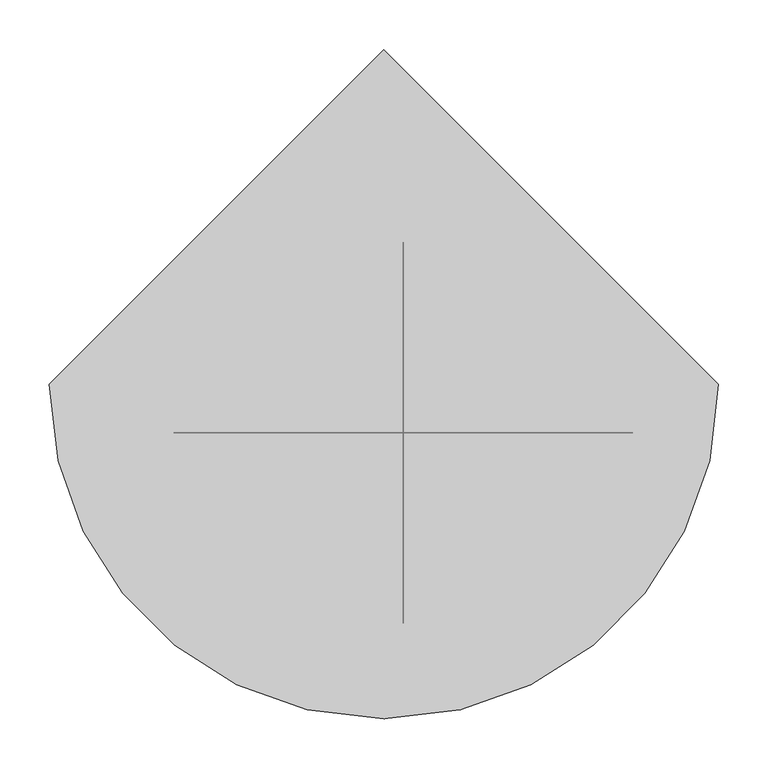
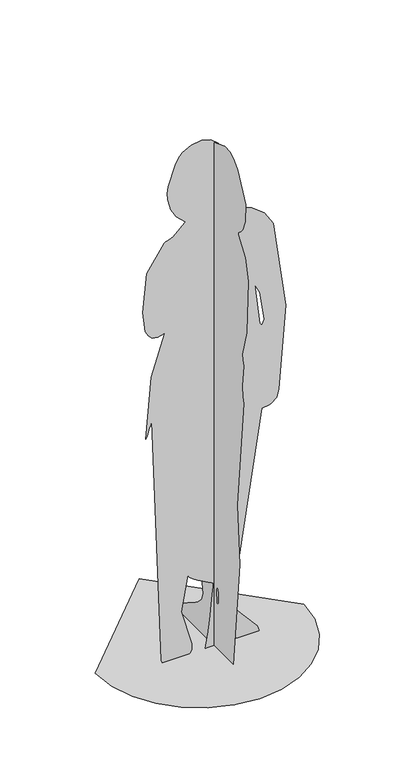
"""IFC4 building model written with IfcOpenShell, lengths in millimetres: proxy geometry, yinyin 25485 : yinyin 25485."""

import ifcopenshell
import ifcopenshell.guid

model = None  # the IFC model being written
_history = None  # IfcOwnerHistory: only IFC2X3 demands one
_inside = {}  # id of a spatial element -> (the spatial element, [elements in it])
_under = {}  # id of a project, library or spatial element -> (it, [spatial elements below it])
_declared = {}  # id of a project -> (the project, [libraries it declares])
_typed = {}  # id of a type object -> (the type object, [elements of that type])
_made_of = {}  # id of a material, layer set ... -> (it, [elements and type objects made of it])


def new_model(schema):
    """Start an empty IFC model of exactly this schema.

    Asked for "IFC4X3", IfcOpenShell would pick the latest addendum, in which some entities
    have other attributes; the version numbers below select the first issue.
    IFC2X3 requires an IfcOwnerHistory on every rooted entity: one is made here for all.
    """
    global model, _history
    if schema == "IFC4X3":
        model = ifcopenshell.file(schema_version=(4, 3, 0, 0))
    else:
        model = ifcopenshell.file(schema=schema)
    _inside.clear()
    _under.clear()
    _declared.clear()
    _typed.clear()
    _made_of.clear()
    _history = None
    if model.schema == "IFC2X3":
        org = make("IfcOrganization", Name="unknown")
        user = make(
            "IfcPersonAndOrganization",
            ThePerson=make("IfcPerson", FamilyName="unknown"),
            TheOrganization=org,
        )
        app = make(
            "IfcApplication",
            ApplicationDeveloper=org,
            Version="unknown",
            ApplicationFullName="unknown",
            ApplicationIdentifier="unknown",
        )
        _history = make(
            "IfcOwnerHistory",
            OwningUser=user,
            OwningApplication=app,
            ChangeAction="ADDED",
            CreationDate=0,
        )
    return model


def make(cls, **values):
    """One entity of the class cls with the attributes given. An attribute that is None is left unset."""
    return model.create_entity(
        cls, **{name: value for name, value in values.items() if value is not None}
    )


def rooted(cls, **values):
    """An entity with a GlobalId (a new one), such as an element, a storey or a relation."""
    return make(cls, GlobalId=ifcopenshell.guid.new(), OwnerHistory=_history, **values)


def si_unit(unit_type, name, prefix=None):
    """IfcSIUnit, for example si_unit("LENGTHUNIT", "METRE", prefix="MILLI")."""
    return make("IfcSIUnit", UnitType=unit_type, Prefix=prefix, Name=name)


def assignment(units):
    """IfcUnitAssignment: the units of a project."""
    return None if units is None else make("IfcUnitAssignment", Units=units)


def point(xyz):
    """IfcCartesianPoint."""
    return None if xyz is None else make("IfcCartesianPoint", Coordinates=xyz)


def direction(xyz):
    """IfcDirection."""
    return None if xyz is None else make("IfcDirection", DirectionRatios=xyz)


def frame(location, z_axis=None, x_axis=None):
    """IfcAxis2Placement3D, a coordinate frame: its origin and axes. An axis left out is left unset."""
    return make(
        "IfcAxis2Placement3D",
        Location=point(location),
        Axis=direction(z_axis),
        RefDirection=direction(x_axis),
    )


def origin():
    """The frame at (0, 0, 0) with its axes left unset."""
    return frame((0.0, 0.0, 0.0))


def place(relative_to, where):
    """IfcLocalPlacement: puts the frame where relative to a parent placement (None: the world)."""
    return make(
        "IfcLocalPlacement", PlacementRelTo=relative_to, RelativePlacement=where
    )


def context(
    kind, dimensions, precision=None, world=None, true_north=None, identifier=None
):
    """IfcGeometricRepresentationContext, for example the 3D "Model" context."""
    return make(
        "IfcGeometricRepresentationContext",
        ContextIdentifier=identifier,
        ContextType=kind,
        CoordinateSpaceDimension=dimensions,
        Precision=precision,
        WorldCoordinateSystem=world,
        TrueNorth=true_north,
    )


def project(units=None, contexts=None):
    """IfcProject with its units and contexts."""
    return rooted(
        "IfcProject",
        Name="project",
        RepresentationContexts=contexts,
        UnitsInContext=assignment(units),
    )


def spatial(cls, under=None, at=None, **own):
    """A site, building, storey or space (cls), placed at a placement, below another one or the project."""
    s = rooted(cls, ObjectPlacement=at, **own)
    if under is not None:
        _under.setdefault(under.id(), (under, []))[1].append(s)
    return s


def point_list(points):
    """IfcCartesianPointList2D or 3D."""
    cls = (
        "IfcCartesianPointList2D" if len(points[0]) == 2 else "IfcCartesianPointList3D"
    )
    return make(cls, CoordList=points)


def triangles(points, corners, closed=None, point_numbers=None):
    """IfcTriangulatedFaceSet: each triangle names its three corners, points numbered from 1."""
    return make(
        "IfcTriangulatedFaceSet",
        Coordinates=point_list(points),
        Closed=closed,
        CoordIndex=corners,
        PnIndex=point_numbers,
    )


def shape(context_of_items, identifier, shape_type, items):
    """IfcShapeRepresentation: the items that make up one representation, for example the "Body"."""
    return make(
        "IfcShapeRepresentation",
        ContextOfItems=context_of_items,
        RepresentationIdentifier=identifier,
        RepresentationType=shape_type,
        Items=items,
    )


def source(mapping_origin, context_of_items, identifier, shape_type, items):
    """IfcRepresentationMap: a shape defined once, which mapped items show again and again."""
    return make(
        "IfcRepresentationMap",
        MappingOrigin=mapping_origin,
        MappedRepresentation=shape(context_of_items, identifier, shape_type, items),
    )


def transform(
    local_origin,
    x_axis=None,
    y_axis=None,
    z_axis=None,
    scale=None,
    scale2=None,
    scale3=None,
    uniform=True,
):
    """IfcCartesianTransformationOperator3D, or its non-uniform kind. x_axis, y_axis, z_axis: its Axis1, 2, 3."""
    if uniform:
        return make(
            "IfcCartesianTransformationOperator3D",
            Axis1=direction(x_axis),
            Axis2=direction(y_axis),
            LocalOrigin=point(local_origin),
            Scale=scale,
            Axis3=direction(z_axis),
        )
    return make(
        "IfcCartesianTransformationOperator3DnonUniform",
        Axis1=direction(x_axis),
        Axis2=direction(y_axis),
        LocalOrigin=point(local_origin),
        Scale=scale,
        Axis3=direction(z_axis),
        Scale2=scale2,
        Scale3=scale3,
    )


def mapped(mapping_source, mapping_target):
    """IfcMappedItem: shows the shape of a source again, moved by a transform."""
    return make(
        "IfcMappedItem", MappingSource=mapping_source, MappingTarget=mapping_target
    )


def made_of(thing, what):
    """Note that an element or type object is made of a material, layer set ...; save() writes the relation."""
    if what is not None:
        _made_of.setdefault(what.id(), (what, []))[1].append(thing)
    return thing


def element(
    cls,
    number,
    at=None,
    inside=None,
    cuts=None,
    type_object=None,
    material=None,
    context=None,
    identifier="Body",
    shape_type=None,
    held_by="IfcProductDefinitionShape",
    body=None,
    shapes=None,
    **own,
):
    """One element of the class cls, such as IfcWall. Its Tag is "e" and its number.

    at: its placement. inside: the storey or other place that contains it. cuts: it is an
    opening in that element (IfcRelVoidsElement). A single representation is given by context,
    identifier, shape_type and body (its items); several are given by shapes. held_by: the class
    of the entity that holds the representations. save() writes the other relations.
    """
    e = rooted(cls, Tag="e%d" % number, ObjectPlacement=at, **own)
    if body is not None:
        shapes = [shape(context, identifier, shape_type, body)]
    if shapes is not None:
        e.Representation = make(held_by, Representations=shapes)
    if inside is not None:
        _inside.setdefault(inside.id(), (inside, []))[1].append(e)
    if cuts is not None:
        rooted(
            "IfcRelVoidsElement", RelatingBuildingElement=cuts, RelatedOpeningElement=e
        )
    if type_object is not None:
        _typed.setdefault(type_object.id(), (type_object, []))[1].append(e)
    return made_of(e, material)


def aggregate(whole, parts):
    """IfcRelAggregates: a whole, such as a stair, and the parts it consists of."""
    return rooted("IfcRelAggregates", RelatingObject=whole, RelatedObjects=parts)


def save(model, path):
    """Write the relations noted so far, then the file.

    IfcRelAggregates (storeys below a building ...), IfcRelContainedInSpatialStructure (elements
    in a storey), IfcRelDefinesByType, IfcRelAssociatesMaterial and IfcRelDeclares: one each for
    every whole, place, type object, material and project.
    """
    for whole, parts in _under.values():
        aggregate(whole, parts)
    for where, things in _inside.values():
        rooted(
            "IfcRelContainedInSpatialStructure",
            RelatedElements=things,
            RelatingStructure=where,
        )
    for kind, things in _typed.values():
        rooted("IfcRelDefinesByType", RelatedObjects=things, RelatingType=kind)
    for what, things in _made_of.values():
        rooted("IfcRelAssociatesMaterial", RelatedObjects=things, RelatingMaterial=what)
    for by, libraries in _declared.values():
        rooted("IfcRelDeclares", RelatingContext=by, RelatedDefinitions=libraries)
    model.write(path)


def entourage_2a7e0e44(model_context):
    return source(origin(), model_context, "Body", "Tessellation", [
        triangles([(19.5612288, -62.516115, 200.054177), (19.5612288, -65.6147495, 206.6420561), (19.5612288, -67.0928433, 208.6188795), (19.5612265, -68.5512254, 210.1580661), (19.5612265, -69.844524, 211.0626257), (19.5612265, -70.8273447, 211.135768), (19.5612265, -72.3676622, 205.9018034), (19.5612265, -74.2961918, 196.3806185), (19.5612265, -75.9136394, 184.6084991), (19.5612265, -76.5207017, 172.6210404), (19.5612265, -75.4180619, 162.4544372), (19.5612265, -71.9064394, 156.1446297), (19.5612288, -65.2864992, 155.7276494), (19.561222, -157.7734002, 0.0), (19.5612197, -193.0714818, 365.6725562), (19.5612197, -178.8732388, 562.9772644), (19.5612197, -217.6589527, 934.2117268), (19.5612197, -211.3346658, 953.6969473), (19.5612197, -209.2266004, 990.3578636), (19.5612197, -217.6589527, 1061.6503143), (19.5612197, -210.505792, 1080.5146425), (19.5612197, -208.859072, 1098.4551172), (19.5612174, -232.5499224, 1186.4916767), (19.5612174, -242.5926415, 1369.1652649), (19.5612197, -225.9702005, 1441.195752), (19.5612197, -184.4141614, 1493.8335274), (19.5612197, -184.4141614, 1502.144648), (19.5612197, -199.7089946, 1513.6221451), (19.5612197, -211.0344297, 1528.1208241), (19.5612197, -224.1337755, 1563.6801361), (19.5612197, -228.7406891, 1624.0425854), (19.5612197, -183.90509, 1715.3903526), (19.561222, -164.1470301, 1737.5990261), (19.561222, -139.3701631, 1750.94981), (19.5612242, -108.0070247, 1752.6), (19.5612288, -48.1992019, 1729.3935677), (19.5612288, -20.4396227, 1708.5970173), (19.5612288, -13.3298936, 1699.5173389), (19.5612288, -7.8875699, 1689.0607098), (19.5612288, -0.7000028, 1662.8370197), (19.5612288, -20.3543195, 1513.0532845), (19.5612288, -18.6669849, 1499.3218552), (19.5612288, 11.1308794, 1439.5698338), (19.5612311, 14.5355749, 1426.8243908), (19.5612288, 1.7224977, 1354.8805264), (19.5612311, 31.6774996, 1150.3032606), (19.5612333, 48.2999633, 1147.5328629), (19.5612333, 62.8445879, 962.6950172), (19.5612356, 95.3969115, 840.0179123), (19.5612356, 94.2716259, 840.4783493), (19.5612356, 92.0029507, 841.6656315), (19.5612356, 89.0270695, 843.2890789), (19.5612356, 85.780102, 845.057939), (19.5612356, 82.698268, 846.6813864), (19.5612356, 80.2176599, 847.8687412), (19.5612356, 78.7744431, 848.3291056), (19.5612379, 129.4411089, 519.2575856), (19.5612356, 115.741936, 386.017608), (19.5612356, 111.0111655, 373.0374773), (19.5612333, 46.365393, 289.3376807), (19.5612311, 27.5485274, 242.7219941), (19.5612288, 11.1591606, 141.8756606), (19.5612311, 19.6101607, 117.1299145), (19.5612311, 40.4985227, 95.464113), (19.5612333, 68.4630586, 75.9257889), (19.5612356, 98.1425106, 57.5627155), (19.5612379, 124.1758143, 39.4220441), (19.5612379, 141.2016192, 20.5520522), (19.5612379, 143.8588244, 0.0), (183.0152098, -49.3669449, 1064.4207121), (167.6047769, -49.3669449, 1163.5493271), (152.5406528, -49.3669449, 1194.6297701), (168.2882199, -49.3669449, 1056.0085802), (175.1435972, -49.3669449, 1046.9906713), (-8.6639288, -49.3669495, 0.0), (-3.1500451, -49.3669495, 32.2482746), (2.0823084, -49.3669495, 69.3733591), (6.8265455, -49.3669495, 108.190362), (10.8761212, -49.3669495, 145.5140468), (14.0244233, -49.3669495, 178.1596922), (16.064901, -49.3669495, 202.9421185), (16.790965, -49.3669495, 216.6765999), (12.1870877, -49.3669495, 219.1461257), (0.3139176, -49.3669495, 225.0791757), (-15.9208339, -49.3669495, 233.4869473), (-33.6094311, -49.3669495, 243.3801843), (-49.8441732, -49.3669495, 253.770157), (-61.7173402, -49.3669495, 263.6679903), (-66.3212244, -49.3669495, 272.0846822), (-87.4455254, -49.3669495, 152.9572698), (-53.4087358, -49.3669495, 31.0045278), (-52.5813699, -49.3669495, 11.0292914), (-59.149233, -49.3669495, 0.0), (-149.3170486, -49.3669495, 0.0), (-152.8115664, -49.3669495, 10.4443548), (-182.6783299, -49.3669495, 842.7883101), (-184.325068, -49.3669495, 839.6736019), (-187.3181266, -49.3669495, 831.6521439), (-191.0743654, -49.3669495, 820.7077538), (-195.0109165, -49.3669495, 808.8246128), (-198.5445671, -49.3669495, 797.9861755), (-201.0923222, -49.3669495, 790.1768412), (-202.0711687, -49.3669495, 787.3802095), (-185.4487277, -49.3669495, 995.1605501), (-141.1222818, -49.3669495, 1130.9104036), (-164.3032524, -49.3669495, 1124.3246864), (-182.0564565, -49.3669495, 1128.1551939), (-195.0603866, -49.3669495, 1140.1605658), (-203.9935441, -49.3669495, 1158.0995871), (-213.1528324, -49.3669495, 1225.1042908), (-199.3008073, -49.3669495, 1355.3133488), (-142.1370091, -49.3669495, 1439.8141502), (-138.3519385, -49.3669495, 1443.9662224), (-126.4535278, -49.3669495, 1446.4888882), (-114.043257, -49.3669495, 1453.0155247), (-76.6084144, -49.3669495, 1487.9363583), (-74.632563, -49.3669495, 1491.0630569), (-103.0904008, -49.3669495, 1516.7510239), (-122.0980524, -49.3669495, 1548.9569069), (-131.6192644, -49.3669495, 1586.7359962), (-132.8111248, -49.3669495, 1607.4201988), (-130.0407362, -49.3669495, 1629.5832355), (-105.4423103, -49.3669495, 1701.5050083), (-96.1691935, -49.3669495, 1717.9445572), (-84.0080717, -49.3669495, 1731.1446236), (-55.2397923, -49.3669495, 1745.9405228), (-21.1277098, -49.3669495, 1752.5937504), (8.678871, -49.3669495, 1743.6800503), (33.6907601, -49.3669495, 1722.8627163), (53.4188279, -49.3669495, 1693.8054783), (75.0667116, -49.3669495, 1625.6246109), (76.0082012, -49.3669495, 1593.8278599), (45.7087471, -49.3669495, 1512.9888988), (45.9664484, -49.3669495, 1502.7510063), (52.5419328, -49.3669495, 1494.1808899), (141.4590436, -49.3669449, 1463.3590794), (183.2079669, -49.3669449, 1431.0789276), (212.1099455, -49.3669449, 1385.7065517), (252.2752991, -49.3669449, 1089.3543646), (230.371894, -49.3669449, 807.1516771), (222.5798733, -49.3669449, 783.138172), (217.6563003, -49.3669449, 776.9216183), (211.9300146, -49.3669449, 771.9938667), (205.4994478, -49.3669449, 768.2337765), (198.4631949, -49.3669449, 765.520134), (174.7039802, -49.3669449, 762.4466297), (101.5479077, -49.3669495, 280.655816), (74.363298, -49.3669495, 138.9321538), (78.7407061, -49.3669495, 117.6130336), (91.1993842, -49.3669495, 97.162465), (159.9730479, -49.3669449, 19.5097603), (166.4327009, -49.3669449, 0.0), (-339.0976521, 0.0001336, 0.0), (-330.1329741, -77.6986367, 0.0), (-304.601829, -149.0525117, 0.0), (-264.5484235, -212.0171641, 0.0), (-212.0172913, -264.548369, 0.0), (-149.0525935, -304.6016654, 0.0), (-77.6987276, -330.1329014, 0.0), (1.42e-05, -339.0975431, 0.000112), (77.6987639, -330.1329014, 0.000112), (149.052648, -304.6016654, 0.000112), (212.0172913, -264.5483145, 0.000112), (264.5485143, -212.0171641, 0.0), (304.6018108, -149.0524572, 0.0), (330.1329741, -77.6985731, 0.0), (339.0976521, 0.000162, 0.0), (-4.4e-05, 339.0977975, 0.0)], [[14, 6, 7], [14, 7, 8], [14, 8, 9], [14, 9, 10], [14, 10, 11], [48, 49, 50], [48, 50, 51], [48, 51, 52], [48, 52, 53], [48, 53, 54], [48, 54, 55], [14, 11, 12], [69, 14, 12], [69, 12, 13], [68, 69, 13], [67, 68, 13], [66, 67, 13], [65, 66, 13], [64, 65, 13], [63, 64, 13], [62, 63, 13], [48, 55, 56], [62, 13, 1], [61, 62, 1], [46, 47, 48], [61, 1, 2], [61, 2, 3], [61, 3, 4], [61, 4, 5], [6, 14, 15], [5, 6, 15], [61, 5, 15], [60, 61, 15], [60, 15, 16], [59, 60, 16], [58, 59, 16], [57, 58, 16], [56, 57, 16], [48, 56, 16], [48, 16, 17], [48, 17, 18], [46, 48, 18], [46, 18, 19], [46, 19, 20], [46, 20, 21], [46, 21, 22], [46, 22, 23], [46, 23, 24], [45, 46, 24], [45, 24, 25], [45, 25, 26], [44, 45, 26], [43, 44, 26], [42, 43, 26], [41, 42, 26], [41, 26, 27], [41, 27, 28], [41, 28, 29], [41, 29, 30], [41, 30, 31], [40, 41, 31], [40, 31, 32], [39, 40, 32], [38, 39, 32], [37, 38, 32], [36, 37, 32], [35, 36, 32], [35, 32, 33], [34, 35, 33], [70, 75, 76], [70, 76, 77], [70, 77, 78], [70, 78, 79], [70, 79, 80], [70, 80, 81], [70, 81, 82], [74, 70, 82], [102, 103, 104], [101, 102, 104], [100, 101, 104], [99, 100, 104], [98, 99, 104], [97, 98, 104], [96, 97, 104], [151, 152, 75], [74, 82, 83], [74, 83, 84], [74, 84, 85], [74, 85, 86], [74, 86, 87], [74, 87, 88], [74, 88, 89], [150, 151, 75], [149, 150, 75], [93, 94, 95], [92, 93, 95], [91, 92, 95], [90, 91, 95], [90, 95, 96], [89, 90, 96], [74, 89, 96], [74, 96, 104], [73, 74, 104], [73, 104, 105], [72, 73, 105], [148, 149, 75], [148, 75, 70], [147, 148, 70], [146, 147, 70], [145, 146, 70], [144, 145, 70], [143, 144, 70], [142, 143, 70], [141, 142, 70], [140, 141, 70], [139, 140, 70], [139, 70, 71], [139, 71, 72], [138, 139, 72], [138, 72, 105], [137, 138, 105], [136, 137, 105], [135, 136, 105], [134, 135, 105], [134, 105, 106], [134, 106, 107], [134, 107, 108], [134, 108, 109], [134, 109, 110], [134, 110, 111], [134, 111, 112], [133, 134, 112], [112, 113, 114], [133, 112, 114], [133, 114, 115], [133, 115, 116], [133, 116, 117], [133, 117, 118], [133, 118, 119], [133, 119, 120], [133, 120, 121], [133, 121, 122], [132, 133, 122], [131, 132, 122], [130, 131, 122], [129, 130, 122], [129, 122, 123], [128, 129, 123], [127, 128, 123], [126, 127, 123], [126, 123, 124], [125, 126, 124], [167, 168, 153], [166, 167, 153], [166, 153, 154], [165, 166, 154], [165, 154, 155], [165, 155, 156], [164, 165, 156], [163, 164, 156], [163, 156, 157], [163, 157, 158], [163, 158, 159], [163, 159, 160], [163, 160, 161], [163, 161, 162]], closed=False),
    ])


if __name__ == "__main__":
    model = new_model("IFC4")
    model_context = context("Model", 3, world=origin())
    ifc_project = project(units=[si_unit("LENGTHUNIT", "METRE", prefix="MILLI")], contexts=[model_context])
    site = spatial("IfcSite", under=ifc_project)
    building = spatial("IfcBuilding", under=site)
    placement = place(None, origin())
    entourage_shape = entourage_2a7e0e44(model_context)
    element("IfcBuildingElementProxy", 1, Name="yinyin 25485 : yinyin 25485", ObjectType="yinyin 25485 : yinyin 25485", at=placement, inside=building, context=model_context, shape_type="MappedRepresentation", body=[
        mapped(entourage_shape, transform((0.0, 0.0, 0.0), x_axis=(1.0, 0.0, 0.0), y_axis=(0.0, 1.0, 0.0), z_axis=(0.0, 0.0, 1.0))),
    ])
    save(model, "model.ifc")

# Revit data of these elements
# Type "yinyin 25485 : yinyin 25485"
#   built-in parameter 1005195 = "RPC-8-FUM5-CKXX-U6B5-E"
#   Height = 0
